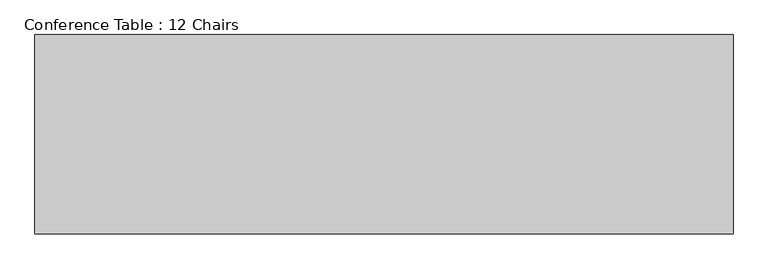
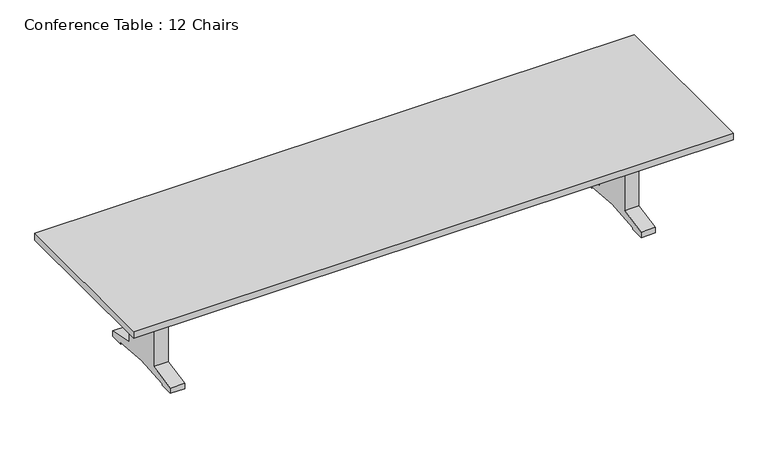
"""IFC4 building model written with IfcOpenShell, lengths in millimetres: furniture geometry, Conference Table : 12 Chairs."""

import ifcopenshell
import ifcopenshell.guid

model = None  # the IFC model being written
_history = None  # IfcOwnerHistory: only IFC2X3 demands one
_inside = {}  # id of a spatial element -> (the spatial element, [elements in it])
_under = {}  # id of a project, library or spatial element -> (it, [spatial elements below it])
_declared = {}  # id of a project -> (the project, [libraries it declares])
_typed = {}  # id of a type object -> (the type object, [elements of that type])
_made_of = {}  # id of a material, layer set ... -> (it, [elements and type objects made of it])


def new_model(schema):
    """Start an empty IFC model of exactly this schema.

    Asked for "IFC4X3", IfcOpenShell would pick the latest addendum, in which some entities
    have other attributes; the version numbers below select the first issue.
    IFC2X3 requires an IfcOwnerHistory on every rooted entity: one is made here for all.
    """
    global model, _history
    if schema == "IFC4X3":
        model = ifcopenshell.file(schema_version=(4, 3, 0, 0))
    else:
        model = ifcopenshell.file(schema=schema)
    _inside.clear()
    _under.clear()
    _declared.clear()
    _typed.clear()
    _made_of.clear()
    _history = None
    if model.schema == "IFC2X3":
        org = make("IfcOrganization", Name="unknown")
        user = make(
            "IfcPersonAndOrganization",
            ThePerson=make("IfcPerson", FamilyName="unknown"),
            TheOrganization=org,
        )
        app = make(
            "IfcApplication",
            ApplicationDeveloper=org,
            Version="unknown",
            ApplicationFullName="unknown",
            ApplicationIdentifier="unknown",
        )
        _history = make(
            "IfcOwnerHistory",
            OwningUser=user,
            OwningApplication=app,
            ChangeAction="ADDED",
            CreationDate=0,
        )
    return model


def make(cls, **values):
    """One entity of the class cls with the attributes given. An attribute that is None is left unset."""
    return model.create_entity(
        cls, **{name: value for name, value in values.items() if value is not None}
    )


def rooted(cls, **values):
    """An entity with a GlobalId (a new one), such as an element, a storey or a relation."""
    return make(cls, GlobalId=ifcopenshell.guid.new(), OwnerHistory=_history, **values)


def si_unit(unit_type, name, prefix=None):
    """IfcSIUnit, for example si_unit("LENGTHUNIT", "METRE", prefix="MILLI")."""
    return make("IfcSIUnit", UnitType=unit_type, Prefix=prefix, Name=name)


def assignment(units):
    """IfcUnitAssignment: the units of a project."""
    return None if units is None else make("IfcUnitAssignment", Units=units)


def point(xyz):
    """IfcCartesianPoint."""
    return None if xyz is None else make("IfcCartesianPoint", Coordinates=xyz)


def direction(xyz):
    """IfcDirection."""
    return None if xyz is None else make("IfcDirection", DirectionRatios=xyz)


def frame(location, z_axis=None, x_axis=None):
    """IfcAxis2Placement3D, a coordinate frame: its origin and axes. An axis left out is left unset."""
    return make(
        "IfcAxis2Placement3D",
        Location=point(location),
        Axis=direction(z_axis),
        RefDirection=direction(x_axis),
    )


def origin():
    """The frame at (0, 0, 0) with its axes left unset."""
    return frame((0.0, 0.0, 0.0))


def place(relative_to, where):
    """IfcLocalPlacement: puts the frame where relative to a parent placement (None: the world)."""
    return make(
        "IfcLocalPlacement", PlacementRelTo=relative_to, RelativePlacement=where
    )


def context(
    kind, dimensions, precision=None, world=None, true_north=None, identifier=None
):
    """IfcGeometricRepresentationContext, for example the 3D "Model" context."""
    return make(
        "IfcGeometricRepresentationContext",
        ContextIdentifier=identifier,
        ContextType=kind,
        CoordinateSpaceDimension=dimensions,
        Precision=precision,
        WorldCoordinateSystem=world,
        TrueNorth=true_north,
    )


def project(units=None, contexts=None):
    """IfcProject with its units and contexts."""
    return rooted(
        "IfcProject",
        Name="project",
        RepresentationContexts=contexts,
        UnitsInContext=assignment(units),
    )


def spatial(cls, under=None, at=None, **own):
    """A site, building, storey or space (cls), placed at a placement, below another one or the project."""
    s = rooted(cls, ObjectPlacement=at, **own)
    if under is not None:
        _under.setdefault(under.id(), (under, []))[1].append(s)
    return s


def polyline(points):
    """IfcPolyline through the points."""
    return make("IfcPolyline", Points=[point(p) for p in points])


def outline(outer, holes=None, kind="AREA"):
    """IfcArbitraryClosedProfileDef: a profile drawn as a closed curve; with holes, ...WithVoids."""
    if holes is None:
        return make("IfcArbitraryClosedProfileDef", ProfileType=kind, OuterCurve=outer)
    return make(
        "IfcArbitraryProfileDefWithVoids",
        ProfileType=kind,
        OuterCurve=outer,
        InnerCurves=holes,
    )


def extrude(swept, where, along, depth):
    """IfcExtrudedAreaSolid: the profile swept, set in the frame where, extruded along a direction by depth."""
    return make(
        "IfcExtrudedAreaSolid",
        SweptArea=swept,
        Position=where,
        ExtrudedDirection=direction(along),
        Depth=depth,
    )


def shape(context_of_items, identifier, shape_type, items):
    """IfcShapeRepresentation: the items that make up one representation, for example the "Body"."""
    return make(
        "IfcShapeRepresentation",
        ContextOfItems=context_of_items,
        RepresentationIdentifier=identifier,
        RepresentationType=shape_type,
        Items=items,
    )


def source(mapping_origin, context_of_items, identifier, shape_type, items):
    """IfcRepresentationMap: a shape defined once, which mapped items show again and again."""
    return make(
        "IfcRepresentationMap",
        MappingOrigin=mapping_origin,
        MappedRepresentation=shape(context_of_items, identifier, shape_type, items),
    )


def transform(
    local_origin,
    x_axis=None,
    y_axis=None,
    z_axis=None,
    scale=None,
    scale2=None,
    scale3=None,
    uniform=True,
):
    """IfcCartesianTransformationOperator3D, or its non-uniform kind. x_axis, y_axis, z_axis: its Axis1, 2, 3."""
    if uniform:
        return make(
            "IfcCartesianTransformationOperator3D",
            Axis1=direction(x_axis),
            Axis2=direction(y_axis),
            LocalOrigin=point(local_origin),
            Scale=scale,
            Axis3=direction(z_axis),
        )
    return make(
        "IfcCartesianTransformationOperator3DnonUniform",
        Axis1=direction(x_axis),
        Axis2=direction(y_axis),
        LocalOrigin=point(local_origin),
        Scale=scale,
        Axis3=direction(z_axis),
        Scale2=scale2,
        Scale3=scale3,
    )


def mapped(mapping_source, mapping_target):
    """IfcMappedItem: shows the shape of a source again, moved by a transform."""
    return make(
        "IfcMappedItem", MappingSource=mapping_source, MappingTarget=mapping_target
    )


def made_of(thing, what):
    """Note that an element or type object is made of a material, layer set ...; save() writes the relation."""
    if what is not None:
        _made_of.setdefault(what.id(), (what, []))[1].append(thing)
    return thing


def element(
    cls,
    number,
    at=None,
    inside=None,
    cuts=None,
    type_object=None,
    material=None,
    context=None,
    identifier="Body",
    shape_type=None,
    held_by="IfcProductDefinitionShape",
    body=None,
    shapes=None,
    **own,
):
    """One element of the class cls, such as IfcWall. Its Tag is "e" and its number.

    at: its placement. inside: the storey or other place that contains it. cuts: it is an
    opening in that element (IfcRelVoidsElement). A single representation is given by context,
    identifier, shape_type and body (its items); several are given by shapes. held_by: the class
    of the entity that holds the representations. save() writes the other relations.
    """
    e = rooted(cls, Tag="e%d" % number, ObjectPlacement=at, **own)
    if body is not None:
        shapes = [shape(context, identifier, shape_type, body)]
    if shapes is not None:
        e.Representation = make(held_by, Representations=shapes)
    if inside is not None:
        _inside.setdefault(inside.id(), (inside, []))[1].append(e)
    if cuts is not None:
        rooted(
            "IfcRelVoidsElement", RelatingBuildingElement=cuts, RelatedOpeningElement=e
        )
    if type_object is not None:
        _typed.setdefault(type_object.id(), (type_object, []))[1].append(e)
    return made_of(e, material)


def aggregate(whole, parts):
    """IfcRelAggregates: a whole, such as a stair, and the parts it consists of."""
    return rooted("IfcRelAggregates", RelatingObject=whole, RelatedObjects=parts)


def save(model, path):
    """Write the relations noted so far, then the file.

    IfcRelAggregates (storeys below a building ...), IfcRelContainedInSpatialStructure (elements
    in a storey), IfcRelDefinesByType, IfcRelAssociatesMaterial and IfcRelDeclares: one each for
    every whole, place, type object, material and project.
    """
    for whole, parts in _under.values():
        aggregate(whole, parts)
    for where, things in _inside.values():
        rooted(
            "IfcRelContainedInSpatialStructure",
            RelatedElements=things,
            RelatingStructure=where,
        )
    for kind, things in _typed.values():
        rooted("IfcRelDefinesByType", RelatedObjects=things, RelatingType=kind)
    for what, things in _made_of.values():
        rooted("IfcRelAssociatesMaterial", RelatedObjects=things, RelatingMaterial=what)
    for by, libraries in _declared.values():
        rooted("IfcRelDeclares", RelatingContext=by, RelatedDefinitions=libraries)
    model.write(path)


def conference_table_12_chairs_3d940985(model_context):
    return source(origin(), model_context, "Body", "SweptSolid", [
        extrude(outline(polyline([(-254.0, 0.0), (-355.6, 0.0), (-355.6, 40.4390459), (-152.4, 79.9371247), (-152.4, 555.8555363), (-457.2, 609.6), (-457.2, 711.2), (457.2, 711.2), (457.2, 609.6), (152.4, 555.8555363), (152.4, 79.9371247), (355.6, 40.4390459), (355.6, 0.0), (254.0, 0.0), (254.0, 12.7), (0.0, 34.9221205), (-254.0, 12.7), (-254.0, 0.0)])), frame((1625.6, 0.0, 0.0), z_axis=(1.0, 0.0, 0.0), x_axis=(0.0, 1.0, 0.0)), (0.0, 0.0, 1.0), 101.6),
        extrude(outline(polyline([(-254.0, 0.0), (-355.6, 0.0), (-355.6, 40.4390459), (-152.4, 79.9371247), (-152.4, 555.8555363), (-457.2, 609.6), (-457.2, 711.2), (457.2, 711.2), (457.2, 609.6), (152.4, 555.8555363), (152.4, 79.9371247), (355.6, 40.4390459), (355.6, 0.0), (254.0, 0.0), (254.0, 12.7), (0.0, 34.9221205), (-254.0, 12.7), (-254.0, 0.0)])), frame((-1727.2, 0.0, 0.0), z_axis=(1.0, 0.0, 0.0), x_axis=(0.0, 1.0, 0.0)), (0.0, 0.0, 1.0), 101.6),
        extrude(outline(polyline([(2133.6, -609.6), (-2133.6, -609.6), (-2133.6, 609.6), (2133.6, 609.6), (2133.6, -609.6)])), frame((0.0, 0.0, 711.2), z_axis=(0.0, 0.0, 1.0), x_axis=(1.0, 0.0, 0.0)), (0.0, 0.0, 1.0), 50.8),
        extrude(outline(polyline([(1625.6, 457.2), (1625.6, 419.1), (-1625.6, 419.1), (-1625.6, 457.2), (1625.6, 457.2)])), frame((0.0, 0.0, 609.6), z_axis=(0.0, 0.0, 1.0), x_axis=(1.0, 0.0, 0.0)), (0.0, 0.0, 1.0), 101.6),
        extrude(outline(polyline([(1625.6, -457.2), (-1625.6, -457.2), (-1625.6, -419.1), (1625.6, -419.1), (1625.6, -457.2)])), frame((0.0, 0.0, 609.6), z_axis=(0.0, 0.0, 1.0), x_axis=(1.0, 0.0, 0.0)), (0.0, 0.0, 1.0), 101.6),
    ])


if __name__ == "__main__":
    model = new_model("IFC4")
    model_context = context("Model", 3, world=origin())
    ifc_project = project(units=[si_unit("LENGTHUNIT", "METRE", prefix="MILLI")], contexts=[model_context])
    site = spatial("IfcSite", under=ifc_project)
    building = spatial("IfcBuilding", under=site)
    placement = place(None, origin())
    conference_table_12_chairs_shape = conference_table_12_chairs_3d940985(model_context)
    element("IfcFurniture", 1, ObjectType="Conference Table : 12 Chairs", at=placement, inside=building, context=model_context, shape_type="MappedRepresentation", body=[
        mapped(conference_table_12_chairs_shape, transform((0.0, 0.0, 0.0), x_axis=(1.0, 0.0, 0.0), y_axis=(0.0, 1.0, 0.0), z_axis=(0.0, 0.0, 1.0))),
    ])
    save(model, "model.ifc")

# Revit data of these elements
# Type "Conference Table : 12 Chairs"
#   Model = "TBL-12CH"
#   Manufacturer = "Acme Furniture"
#   Type Mark = "TB-2"
#   Cost = 9250
#   Width = 4' - 0"
#   Length = 14' - 0"
#   Height = 2' - 6"
#   Number of Chairs = 12
#   Number Of Chairs One Side = 5
#   Top = Mahogany
#   Legs and Supports = Mahogany
#   Default Elevation = 0
# Element 1 (IfcFurniture, "Conference Table : 12 Chairs")
#   Materials on its faces: "Mahogany"
# Materials
#   "Mahogany": class "Wood", colour RGB 102 51 32, transparency 0, Description = "Swietenia Macrophylla", Cost = 0
